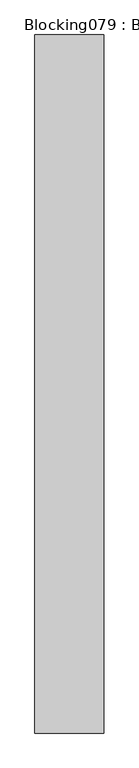
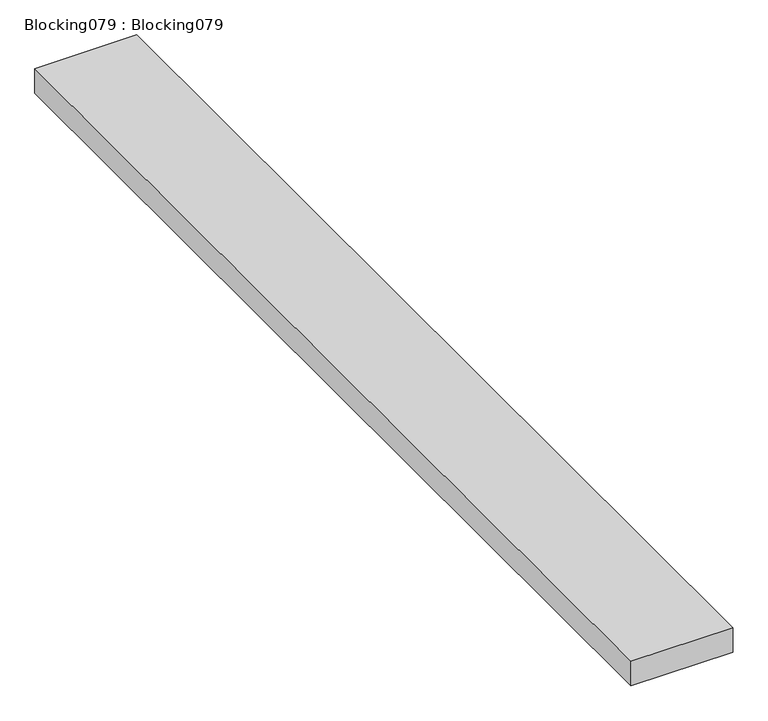
"""IFC4 building model written with IfcOpenShell, lengths in millimetres: proxy geometry, Blocking079 : Blocking079."""

from ifc_helpers import new_model, si_unit, frame, origin, place, context, project, spatial, polyline, outline, extrude, source, transform, mapped, element, save


def blocking079_blocking079_be19e32f(model_context):
    return source(origin(), model_context, "Body", "SweptSolid", [
        extrude(outline(polyline([(-4601.0538825, 934.6593428), (-4404.2038825, 934.6593428), (-4404.2038825, -1065.3406572), (-4601.0538825, -1065.3406572), (-4601.0538825, 934.6593428)])), frame((0.0, 0.0, 40131.746), z_axis=(0.0, 0.0, 1.0), x_axis=(1.0, 0.0, 0.0)), (0.0, 0.0, 1.0), 50.8),
    ])


if __name__ == "__main__":
    model = new_model("IFC4")
    model_context = context("Model", 3, world=origin())
    ifc_project = project(units=[si_unit("LENGTHUNIT", "METRE", prefix="MILLI")], contexts=[model_context])
    site = spatial("IfcSite", under=ifc_project)
    building = spatial("IfcBuilding", under=site)
    placement = place(None, origin())
    blocking079_blocking079_shape = blocking079_blocking079_be19e32f(model_context)
    element("IfcBuildingElementProxy", 1, Name="Blocking079 : Blocking079", ObjectType="Blocking079 : Blocking079", at=placement, inside=building, context=model_context, shape_type="MappedRepresentation", body=[
        mapped(blocking079_blocking079_shape, transform((0.0, 0.0, 0.0), x_axis=(1.0, 0.0, 0.0), y_axis=(0.0, 1.0, 0.0), z_axis=(0.0, 0.0, 1.0))),
    ])
    save(model, "model.ifc")

# Revit data of these elements
# Type "Blocking079 : Blocking079"
#   NameOverride = "Blocking079"
# Element 1 (IfcBuildingElementProxy, "Blocking079 : Blocking079")
#   Materials on its faces: "WOOD BLOCKING AS REQUIRED"
# Materials
#   "WOOD BLOCKING AS REQUIRED": class "Unassigned", colour RGB 166 124 85, transparency 0, Cost = 0
